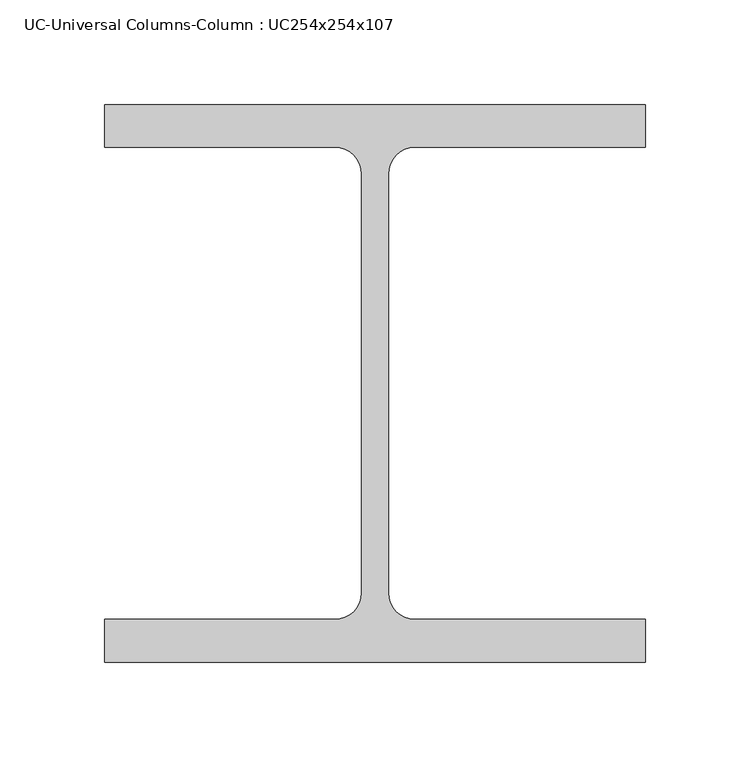
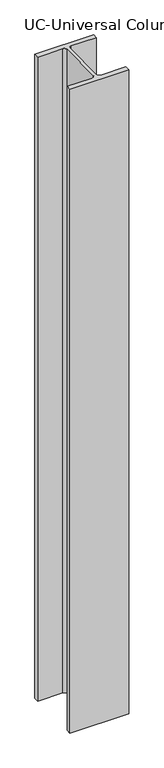
"""IFC4 building model written with IfcOpenShell, lengths in millimetres: column geometry, UC-Universal Columns-Column : UC254x254x107."""

from ifc_helpers import new_model, si_unit, point, frame, frame_2d, origin, place, context, project, spatial, polyline, circle_curve, trimmed, segment, composite_curve, outline, extrude, source, transform, mapped, element, save


def uc_universal_columns_column_uc254x254x107_3d380806(model_context):
    return source(origin(), model_context, "Body", "SweptSolid", [
        extrude(outline(composite_curve([segment(polyline([(129.4, 133.35), (129.4, 112.85), (19.1, 112.85)]), True, "CONTINUOUS"), segment(trimmed(circle_curve(frame_2d((19.1, 100.15)), 12.7), [point((19.1, 112.85))], [point((6.4, 100.15))], True, "CARTESIAN"), True, "CONTINUOUS"), segment(polyline([(6.4, 100.15), (6.4, -100.15)]), True, "CONTINUOUS"), segment(trimmed(circle_curve(frame_2d((19.1, -100.15)), 12.7), [point((6.4, -100.15))], [point((19.1, -112.85))], True, "CARTESIAN"), True, "CONTINUOUS"), segment(polyline([(19.1, -112.85), (129.4, -112.85), (129.4, -133.35), (-129.4, -133.35), (-129.4, -112.85), (-19.1, -112.85)]), True, "CONTINUOUS"), segment(trimmed(circle_curve(frame_2d((-19.1, -100.15)), 12.7), [point((-19.1, -112.85))], [point((-6.4, -100.15))], True, "CARTESIAN"), True, "CONTINUOUS"), segment(polyline([(-6.4, -100.15), (-6.4, 100.15)]), True, "CONTINUOUS"), segment(trimmed(circle_curve(frame_2d((-19.1, 100.15)), 12.7), [point((-6.4, 100.15))], [point((-19.1, 112.85))], True, "CARTESIAN"), True, "CONTINUOUS"), segment(polyline([(-19.1, 112.85), (-129.4, 112.85), (-129.4, 133.35), (129.4, 133.35)]), True, "CONTINUOUS")], self_intersect=False)), frame((0.0, 0.0, 3000.0), z_axis=(0.0, 0.0, 1.0), x_axis=(1.0, 0.0, 0.0)), (0.0, 0.0, 1.0), 3000.0),
    ])


if __name__ == "__main__":
    model = new_model("IFC4")
    model_context = context("Model", 3, world=origin())
    ifc_project = project(units=[si_unit("LENGTHUNIT", "METRE", prefix="MILLI")], contexts=[model_context])
    site = spatial("IfcSite", under=ifc_project)
    building = spatial("IfcBuilding", under=site)
    placement = place(None, origin())
    uc_universal_columns_column_uc254x254x107_shape = uc_universal_columns_column_uc254x254x107_3d380806(model_context)
    element("IfcColumn", 1, ObjectType="UC-Universal Columns-Column : UC254x254x107", at=placement, inside=building, context=model_context, shape_type="MappedRepresentation", body=[
        mapped(uc_universal_columns_column_uc254x254x107_shape, transform((0.0, 0.0, 0.0), x_axis=(1.0, 0.0, 0.0), y_axis=(0.0, 1.0, 0.0), z_axis=(0.0, 0.0, 1.0))),
    ])
    save(model, "model.ifc")

# Revit data of these elements
# Project information
#   ModelCreatedBy = "???"
#   ModelCreationDate = "???"
#   ModelReference = "???"
#   RevitVersion = "???"
#   BIM Coordinator = "???"
#   Project Engineer = "???"
#   Organization Name = "Whitby Wood"
#   Organization Description = "WW"
#   NBLProjectId = "6556f746-0255-4f5f-a425-a0b7f3ea3386"
#   Project Issue Date = "Issue Date"
#   Project Status = "Project Status"
#   Client Name = "Owner"
#   Project Address = "Enter address here"
#   Project Name = "Project Name"
#   Project Number = "P12345"
#   Extensions.Parameters = "2016.5"
#   Project Name 2 = "Project Name"
# Type "UC-Universal Columns-Column : UC254x254x107"
#   Section Name Key = "UC254x254x107"
#   Width = 25.88 cm
#   Web Thickness = 1.28 cm
#   Web Fillet = 1.27 cm
#   Warping Constant = 898000.0 cm⁶
#   Torsional Moment of Inertia = 172.00 cm⁴
#   Section Area = 136.0 cm²
#   Plastic Modulus weak axis = 697.0 cm³
#   Plastic Modulus strong axis = 1485.0 cm³
#   Nominal Weight = 107.10 kgf/m
#   Moment of Inertia weak axis = 5928.00 cm⁴
#   Moment of Inertia strong axis = 17510.00 cm⁴
#   Height = 26.67 cm
#   Flange Thickness = 2.05 cm
#   Elastic Modulus weak axis = 458.0 cm³
#   Elastic Modulus strong axis = 1313.0 cm³
#   Centroid Vertical = 13.335 cm
#   Centroid Horizontal = 12.94 cm
#   Bolt Spacing = 14.0 cm
#   Structural Material [instance default] = Metal - Steel 43-275
#   Type Comments = ""
#   Assembly Code = ""
# Element 1 (IfcColumn, "UC-Universal Columns-Column : UC254x254x107")
#   Structural Material = Metal - Steel
#   Materials on its faces: "Metal - Steel"
# Materials
#   "Metal - Steel 43-275": class "Metal", colour RGB 255 128 0, transparency 0, Cost = 0
#   "Metal - Steel": class "Metal", colour RGB 255 128 0, transparency 0, Cost = 0
